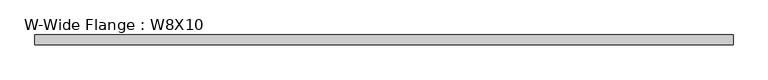
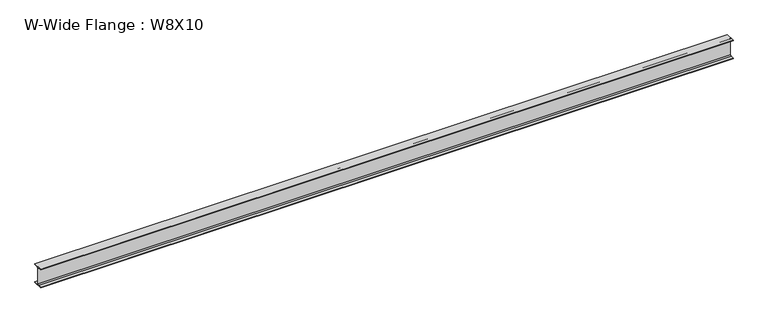
"""IFC4 building model written with IfcOpenShell, lengths in millimetres: beam geometry, W-Wide Flange : W8X10."""

from ifc_helpers import new_model, si_unit, point, frame, frame_2d, origin, place, context, project, spatial, polyline, circle_curve, trimmed, segment, composite_curve, outline, extrude, source, transform, mapped, element, save


def w_wide_flange_w8x10_f1f82eed(model_context):
    return source(origin(), model_context, "Body", "SweptSolid", [
        extrude(outline(composite_curve([segment(polyline([(50.038, -94.996), (50.038, -100.203), (-50.038, -100.203), (-50.038, -94.996), (-14.4145, -94.996)]), True, "CONTINUOUS"), segment(trimmed(circle_curve(frame_2d((-14.4145, -82.7405)), 12.2555), [point((-14.4145, -94.996))], [point((-2.159, -82.7405))], True, "CARTESIAN"), True, "CONTINUOUS"), segment(polyline([(-2.159, -82.7405), (-2.159, 82.7405)]), True, "CONTINUOUS"), segment(trimmed(circle_curve(frame_2d((-14.4145, 82.7405)), 12.2555), [point((-2.159, 82.7405))], [point((-14.4145, 94.996))], True, "CARTESIAN"), True, "CONTINUOUS"), segment(polyline([(-14.4145, 94.996), (-50.038, 94.996), (-50.038, 100.203), (50.038, 100.203), (50.038, 94.996), (14.4145, 94.996)]), True, "CONTINUOUS"), segment(trimmed(circle_curve(frame_2d((14.4145, 82.7405)), 12.2555), [point((14.4145, 94.996))], [point((2.159, 82.7405))], True, "CARTESIAN"), True, "CONTINUOUS"), segment(polyline([(2.159, 82.7405), (2.159, -82.7405)]), True, "CONTINUOUS"), segment(trimmed(circle_curve(frame_2d((14.4145, -82.7405)), 12.2555), [point((2.159, -82.7405))], [point((14.4145, -94.996))], True, "CARTESIAN"), True, "CONTINUOUS"), segment(polyline([(14.4145, -94.996), (50.038, -94.996)]), True, "CONTINUOUS")], self_intersect=False)), frame((-3555.238, 0.0, 0.0), z_axis=(1.0, 0.0, 0.0), x_axis=(0.0, 1.0, 0.0)), (0.0, 0.0, 1.0), 7110.476),
    ])


if __name__ == "__main__":
    model = new_model("IFC4")
    model_context = context("Model", 3, world=origin())
    ifc_project = project(units=[si_unit("LENGTHUNIT", "METRE", prefix="MILLI")], contexts=[model_context])
    site = spatial("IfcSite", under=ifc_project)
    building = spatial("IfcBuilding", under=site)
    placement = place(None, origin())
    w_wide_flange_w8x10_shape = w_wide_flange_w8x10_f1f82eed(model_context)
    element("IfcBeam", 1, ObjectType="W-Wide Flange : W8X10", at=placement, inside=building, context=model_context, shape_type="MappedRepresentation", body=[
        mapped(w_wide_flange_w8x10_shape, transform((0.0, 0.0, 0.0), x_axis=(1.0, 0.0, 0.0), y_axis=(0.0, 1.0, 0.0), z_axis=(0.0, 0.0, 1.0))),
    ])
    save(model, "model.ifc")

# Revit data of these elements
# Type "W-Wide Flange : W8X10"
#   Assembly Code = "B10"
#   W = 10
#   Length [instance default] = 5' - 0"
#   bf = 0' - 3.94"
#   d = 0' - 7.89"
#   k = 0' - 0 11/16"
#   k2 = 0' - 0.4825"
#   tf = 0' - 0.205"
#   tw = 0' - 0.17"
#   A = 0.0205556 SF
#   Structural Material [instance default] = Steel ASTM A992
# Element 1 (IfcBeam, "W-Wide Flange : W8X10")
#   Structural Material = none
# Materials
#   "Steel ASTM A992": class "Metal", colour RGB 189 187 185, transparency 0, Description = "Structural steel 50ksi", Cost = 0
